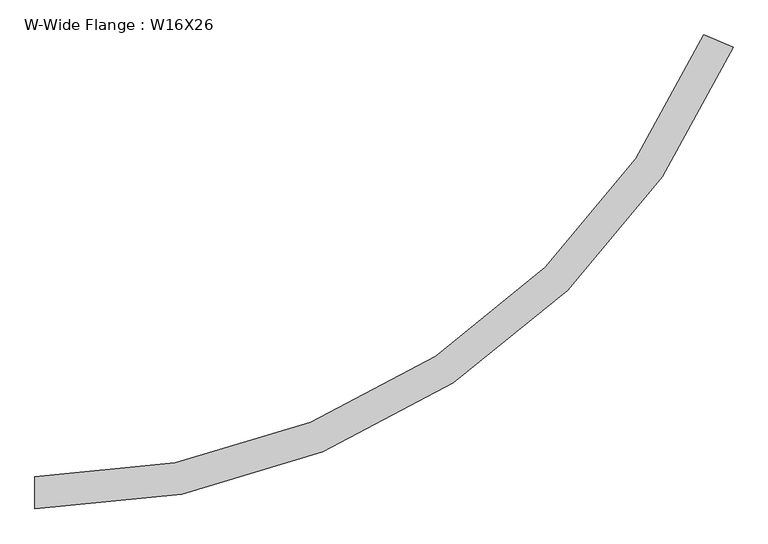
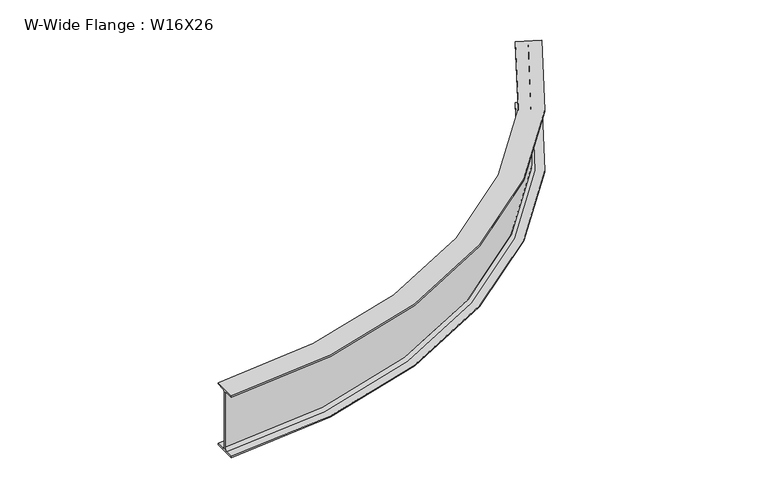
"""IFC4 building model written with IfcOpenShell, lengths in millimetres: beam geometry, W-Wide Flange : W16X26."""

from ifc_helpers import new_model, si_unit, point, frame, origin, place, context, project, spatial, polyline, circle_curve, ellipse_curve, trimmed, source, transform, mapped, element, save
from ifc_brep_helpers import plane_surface, cylinder_surface, revolved_surface, advanced_brep


def w_wide_flange_w16x26_8902d683(model_context):
    return source(origin(), model_context, "Body", "AdvancedBrep", [
        advanced_brep(
        [(3047.7966024, 1943.1127488, -190.5496094), (3047.7966024, 1943.1127488, -199.2808594), (2919.3102414, 1997.9520143, -199.2808594), (2919.3102414, 1997.9520143, -190.5496094), (2963.842446, 1978.9452234, -190.5496094), (2980.6332773, 1971.7787285, -172.2933594), (2980.6332773, 1971.7787285, 172.2933594), (2963.842446, 1978.9452234, 190.5496094), (2919.3102414, 1997.9520143, 190.5496094), (2919.3102414, 1997.9520143, 199.2808594), (3047.7966024, 1943.1127488, 199.2808594), (3047.7966024, 1943.1127488, 190.5496094), (3003.2643977, 1962.1195397, 190.5496094), (2986.4735664, 1969.2860346, 172.2933594), (2986.4735664, 1969.2860346, -172.2933594), (3003.2643977, 1962.1195397, -190.5496094), (0.0, -69.85, -190.5496094), (0.0, -21.43125, -190.5496094), (0.0, -3.175, -172.2933594), (0.0, -3.175, 172.2933594), (0.0, -21.43125, 190.5496094), (0.0, -69.85, 190.5496094), (0.0, -69.85, 199.2808594), (0.0, 69.85, 199.2808594), (0.0, 69.85, 190.5496094), (0.0, 21.43125, 190.5496094), (0.0, 3.175, 172.2933594), (0.0, 3.175, -172.2933594), (0.0, 21.43125, -190.5496094), (0.0, 69.85, -190.5496094), (0.0, 69.85, -199.2808594), (0.0, -69.85, -199.2808594)],
        [
            (0, 1),
            (1, 2),
            (2, 3),
            (3, 4),
            (4, 5, circle_curve(frame((2963.842446, 1978.9452234, -172.2933594), z_axis=(-0.3925502179509604, -0.9197305727149955, 0.0), x_axis=(-0.9197305727149955, 0.3925502179509604, 0.0)), 18.25625)),
            (5, 6),
            (6, 7, circle_curve(frame((2963.842446, 1978.9452234, 172.2933594), z_axis=(-0.3925502179509604, -0.9197305727149955, 0.0), x_axis=(-0.9197305727149955, 0.3925502179509604, 0.0)), 18.25625)),
            (7, 8),
            (8, 9),
            (9, 10),
            (10, 11),
            (11, 12),
            (12, 13, circle_curve(frame((3003.2643977, 1962.1195397, 172.2933594), z_axis=(-0.3925502179509604, -0.9197305727149955, 0.0), x_axis=(-0.9197305727149955, 0.3925502179509604, 0.0)), 18.25625)),
            (13, 14),
            (14, 15, circle_curve(frame((3003.2643977, 1962.1195397, -172.2933594), z_axis=(-0.3925502179509604, -0.9197305727149955, 0.0), x_axis=(-0.9197305727149955, 0.3925502179509604, 0.0)), 18.25625)),
            (15, 0),
            (16, 17),
            (17, 18, circle_curve(frame((0.0, -21.43125, -172.2933594), z_axis=(1.0, 0.0, 0.0), x_axis=(0.0, 1.0, 0.0)), 18.25625)),
            (18, 19),
            (19, 20, circle_curve(frame((0.0, -21.43125, 172.2933594), z_axis=(1.0, 0.0, 0.0), x_axis=(0.0, 1.0, 0.0)), 18.25625)),
            (20, 21),
            (21, 22),
            (22, 23),
            (23, 24),
            (24, 25),
            (25, 26, circle_curve(frame((0.0, 21.43125, 172.2933594), z_axis=(1.0, 0.0, 0.0), x_axis=(0.0, 1.0, 0.0)), 18.25625)),
            (26, 27),
            (27, 28, circle_curve(frame((0.0, 21.43125, -172.2933594), z_axis=(1.0, 0.0, 0.0), x_axis=(0.0, 1.0, 0.0)), 18.25625)),
            (28, 29),
            (29, 30),
            (30, 31),
            (31, 16),
            (15, 17, circle_curve(frame((0.0, 3243.9428571, -190.5496094), z_axis=(0.0, 0.0, -1.0), x_axis=(-1.0, 0.0, 0.0)), 3265.3741071)),
            (16, 0, circle_curve(frame((0.0, 3243.9428571, -190.5496094), z_axis=(0.0, 0.0, 1.0), x_axis=(-1.0, 0.0, 0.0)), 3313.7928571)),
            (14, 18, circle_curve(frame((0.0, 3243.9428571, -172.2933594), z_axis=(0.0, 0.0, -1.0), x_axis=(-1.0, 0.0, 0.0)), 3247.1178571)),
            (13, 19, circle_curve(frame((0.0, 3243.9428571, 172.2933594), z_axis=(0.0, 0.0, -1.0), x_axis=(-1.0, 0.0, 0.0)), 3247.1178571)),
            (12, 20, circle_curve(frame((0.0, 3243.9428571, 190.5496094), z_axis=(0.0, 0.0, -1.0), x_axis=(-1.0, 0.0, 0.0)), 3265.3741071)),
            (11, 21, circle_curve(frame((0.0, 3243.9428571, 190.5496094), z_axis=(0.0, 0.0, -1.0), x_axis=(-1.0, 0.0, 0.0)), 3313.7928571)),
            (10, 22, circle_curve(frame((0.0, 3243.9428571, 199.2808594), z_axis=(0.0, 0.0, -1.0), x_axis=(-1.0, 0.0, 0.0)), 3313.7928571)),
            (9, 23, circle_curve(frame((0.0, 3243.9428571, 199.2808594), z_axis=(0.0, 0.0, -1.0), x_axis=(-1.0, 0.0, 0.0)), 3174.0928571)),
            (8, 24, circle_curve(frame((0.0, 3243.9428571, 190.5496094), z_axis=(0.0, 0.0, -1.0), x_axis=(-1.0, 0.0, 0.0)), 3174.0928571)),
            (7, 25, circle_curve(frame((0.0, 3243.9428571, 190.5496094), z_axis=(0.0, 0.0, -1.0), x_axis=(-1.0, 0.0, 0.0)), 3222.5116071)),
            (6, 26, circle_curve(frame((0.0, 3243.9428571, 172.2933594), z_axis=(0.0, 0.0, -1.0), x_axis=(-1.0, 0.0, 0.0)), 3240.7678571)),
            (5, 27, circle_curve(frame((0.0, 3243.9428571, -172.2933594), z_axis=(0.0, 0.0, -1.0), x_axis=(-1.0, 0.0, 0.0)), 3240.7678571)),
            (4, 28, circle_curve(frame((0.0, 3243.9428571, -190.5496094), z_axis=(0.0, 0.0, -1.0), x_axis=(-1.0, 0.0, 0.0)), 3222.5116071)),
            (3, 29, circle_curve(frame((0.0, 3243.9428571, -190.5496094), z_axis=(0.0, 0.0, -1.0), x_axis=(-1.0, 0.0, 0.0)), 3174.0928571)),
            (2, 30, circle_curve(frame((0.0, 3243.9428571, -199.2808594), z_axis=(0.0, 0.0, -1.0), x_axis=(-1.0, 0.0, 0.0)), 3174.0928571)),
            (1, 31, circle_curve(frame((0.0, 3243.9428571, -199.2808594), z_axis=(0.0, 0.0, -1.0), x_axis=(-1.0, 0.0, 0.0)), 3313.7928571)),
        ],
        [
            plane_surface(frame((2983.5534219, 1970.5323816, 0.0), z_axis=(0.39255021795095457, 0.9197305727149979, 0.0), x_axis=(0.0, 0.0, 1.0))),
            plane_surface(frame((0.0, 0.0, 0.0), z_axis=(-1.0, 0.0, 0.0), x_axis=(0.0, 0.0, 1.0))),
            plane_surface(frame((0.0, 3243.9428571, -190.5496094), z_axis=(0.0, 0.0, 1.0), x_axis=(-1.0, 0.0, 0.0))),
            revolved_surface(trimmed(ellipse_curve(frame((-3265.3741071, 3243.9428571, -172.2933594), z_axis=(0.0, 1.0, 0.0), x_axis=(1.0, 0.0, 0.0)), 18.25625, 18.25625), [point((-3247.1178571, 3243.9428571, -172.2933594))], [point((-3265.3741071, 3243.9428571, -190.5496094))], True, "CARTESIAN"), (0.0, 3243.9428571, 0.0), (0.0, 0.0, -1.0)),
            cylinder_surface(frame((0.0, 3243.9428571, 0.0), z_axis=(0.0, 0.0, -1.0), x_axis=(-1.0, 0.0, 0.0)), 3247.1178571),
            revolved_surface(trimmed(ellipse_curve(frame((-3265.3741071, 3243.9428571, 172.2933594), z_axis=(0.0, 1.0, 0.0), x_axis=(1.0, 0.0, 0.0)), 18.25625, 18.25625), [point((-3265.3741071, 3243.9428571, 190.5496094))], [point((-3247.1178571, 3243.9428571, 172.2933594))], True, "CARTESIAN"), (0.0, 3243.9428571, 0.0), (0.0, 0.0, -1.0)),
            plane_surface(frame((0.0, 3243.9428571, 190.5496094), z_axis=(0.0, 0.0, -1.0), x_axis=(-1.0, 0.0, 0.0))),
            cylinder_surface(frame((0.0, 3243.9428571, 0.0), z_axis=(0.0, 0.0, -1.0), x_axis=(-1.0, 0.0, 0.0)), 3313.7928571),
            plane_surface(frame((0.0, 3243.9428571, 199.2808594), z_axis=(0.0, 0.0, 1.0), x_axis=(-1.0, 0.0, 0.0))),
            revolved_surface(polyline([(-3174.0928571, 3243.9428571, 190.5496094), (-3174.0928571, 3243.9428571, 199.2808594)]), (0.0, 3243.9428571, 0.0), (0.0, 0.0, -1.0)),
            revolved_surface(trimmed(ellipse_curve(frame((-3222.5116071, 3243.9428571, 172.2933594), z_axis=(0.0, 1.0, 0.0), x_axis=(1.0, 0.0, 0.0)), 18.25625, 18.25625), [point((-3240.7678571, 3243.9428571, 172.2933594))], [point((-3222.5116071, 3243.9428571, 190.5496094))], True, "CARTESIAN"), (0.0, 3243.9428571, 0.0), (0.0, 0.0, -1.0)),
            revolved_surface(polyline([(-3240.7678571, 3243.9428571, -172.2933594), (-3240.7678571, 3243.9428571, 172.2933594)]), (0.0, 3243.9428571, 0.0), (0.0, 0.0, -1.0)),
            revolved_surface(trimmed(ellipse_curve(frame((-3222.5116071, 3243.9428571, -172.2933594), z_axis=(0.0, 1.0, 0.0), x_axis=(1.0, 0.0, 0.0)), 18.25625, 18.25625), [point((-3222.5116071, 3243.9428571, -190.5496094))], [point((-3240.7678571, 3243.9428571, -172.2933594))], True, "CARTESIAN"), (0.0, 3243.9428571, 0.0), (0.0, 0.0, -1.0)),
            revolved_surface(polyline([(-3174.0928571, 3243.9428571, -199.2808594), (-3174.0928571, 3243.9428571, -190.5496094)]), (0.0, 3243.9428571, 0.0), (0.0, 0.0, -1.0)),
            plane_surface(frame((0.0, 3243.9428571, -199.2808594), z_axis=(0.0, 0.0, -1.0), x_axis=(-1.0, 0.0, 0.0))),
        ],
        [
            (0, [[1, 2, 3, 4, 5, 6, 7, 8, 9, 10, 11, 12, 13, 14, 15, 16]]),
            (1, [[17, 18, 19, 20, 21, 22, 23, 24, 25, 26, 27, 28, 29, 30, 31, 32]]),
            (2, [[33, -17, 34, -16]]),
            (3, [[35, -18, -33, -15]]),
            (4, [[36, -19, -35, -14]]),
            (5, [[37, -20, -36, -13]]),
            (6, [[38, -21, -37, -12]]),
            (7, [[39, -22, -38, -11]]),
            (8, [[40, -23, -39, -10]]),
            (9, [[41, -24, -40, -9]]),
            (6, [[42, -25, -41, -8]]),
            (10, [[43, -26, -42, -7]]),
            (11, [[44, -27, -43, -6]]),
            (12, [[45, -28, -44, -5]]),
            (2, [[46, -29, -45, -4]]),
            (13, [[47, -30, -46, -3]]),
            (14, [[48, -31, -47, -2]]),
            (7, [[-34, -32, -48, -1]]),
        ],
    ),
    ])


if __name__ == "__main__":
    model = new_model("IFC4")
    model_context = context("Model", 3, world=origin())
    ifc_project = project(units=[si_unit("LENGTHUNIT", "METRE", prefix="MILLI")], contexts=[model_context])
    site = spatial("IfcSite", under=ifc_project)
    building = spatial("IfcBuilding", under=site)
    placement = place(None, origin())
    w_wide_flange_w16x26_shape = w_wide_flange_w16x26_8902d683(model_context)
    element("IfcBeam", 1, ObjectType="W-Wide Flange : W16X26", at=placement, inside=building, context=model_context, shape_type="MappedRepresentation", body=[
        mapped(w_wide_flange_w16x26_shape, transform((0.0, 0.0, 0.0), x_axis=(1.0, 0.0, 0.0), y_axis=(0.0, 1.0, 0.0), z_axis=(0.0, 0.0, 1.0))),
    ])
    save(model, "model.ifc")

# Revit data of these elements
# Type "W-Wide Flange : W16X26"
#   Assembly Code = "B10"
#   W = 26
#   Start Extension Calculation [instance default] = 10' - 0"
#   Start Extension [instance default] = -0' - 0 1/2"
#   End Extension Calculation [instance default] = 10' - 0"
#   End Extension [instance default] = -0' - 0 1/2"
#   Length [instance default] = 5' - 0"
#   bf = 0' - 5 1/2"
#   d = 1' - 3 177/256"
#   k = 0' - 1 1/16"
#   k2 = 0' - 0 23/32"
#   tf = 0' - 0 11/32"
#   tw = 0' - 0 1/4"
#   A = 0.05 SF
#   Beam Material [instance default] = Metal - Steel - ASTM A992
# Element 1 (IfcBeam, "W-Wide Flange : W16X26")
#   Materials on its faces: "Metal - Steel - ASTM A992"
# Materials
#   "Metal - Steel - ASTM A992": class "Metal", colour RGB 128 0 0, transparency 0
